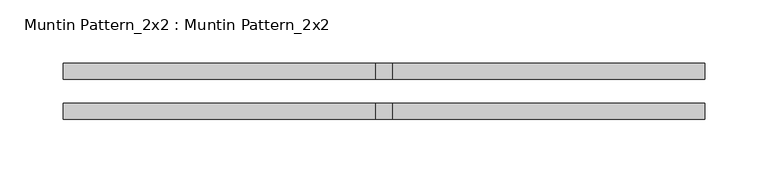
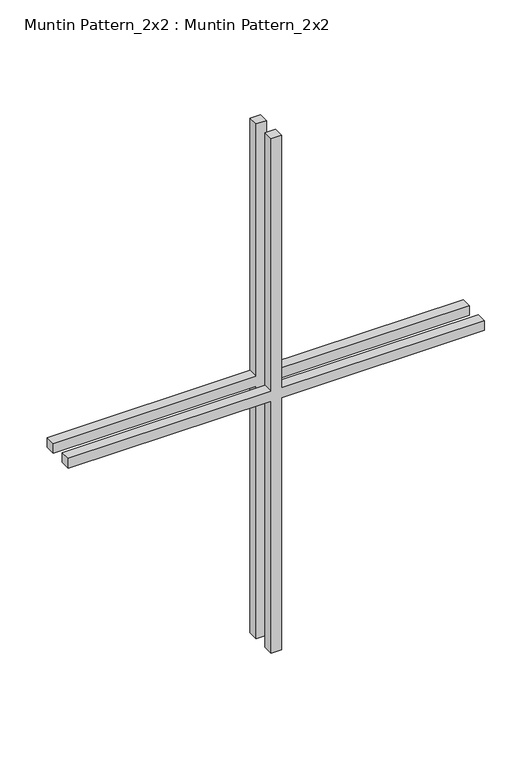
"""IFC4 building model written with IfcOpenShell, lengths in millimetres: proxy geometry, Muntin Pattern_2x2 : Muntin Pattern_2x2."""

from ifc_helpers import new_model, si_unit, frame, origin, place, context, project, spatial, polyline, outline, extrude, source, transform, mapped, element, save


def muntin_pattern_2x2_muntin_pattern_2x2_3eb6ceea(model_context):
    return source(origin(), model_context, "Body", "SweptSolid", [
        extrude(outline(polyline([(338.1375, -6.35), (338.1375, -254.0), (325.4375, -254.0), (325.4375, -6.35), (0.0, -6.35), (0.0, 6.35), (325.4375, 6.35), (325.4375, 254.0), (338.1375, 254.0), (338.1375, 6.35), (663.575, 6.35), (663.575, -6.35), (338.1375, -6.35)])), frame((0.0, -22.225, 0.0), z_axis=(0.0, 1.0, 0.0), x_axis=(0.0, 0.0, 1.0)), (0.0, 0.0, 1.0), 12.7),
        extrude(outline(polyline([(338.1375, -6.35), (338.1375, -254.0), (325.4375, -254.0), (325.4375, -6.35), (0.0, -6.35), (0.0, 6.35), (325.4375, 6.35), (325.4375, 254.0), (338.1375, 254.0), (338.1375, 6.35), (663.575, 6.35), (663.575, -6.35), (338.1375, -6.35)])), frame((0.0, 9.525, 0.0), z_axis=(0.0, 1.0, 0.0), x_axis=(0.0, 0.0, 1.0)), (0.0, 0.0, 1.0), 12.7),
    ])


if __name__ == "__main__":
    model = new_model("IFC4")
    model_context = context("Model", 3, world=origin())
    ifc_project = project(units=[si_unit("LENGTHUNIT", "METRE", prefix="MILLI")], contexts=[model_context])
    site = spatial("IfcSite", under=ifc_project)
    building = spatial("IfcBuilding", under=site)
    placement = place(None, origin())
    muntin_pattern_2x2_muntin_pattern_2x2_shape = muntin_pattern_2x2_muntin_pattern_2x2_3eb6ceea(model_context)
    element("IfcBuildingElementProxy", 1, Name="Muntin Pattern_2x2 : Muntin Pattern_2x2", ObjectType="Muntin Pattern_2x2 : Muntin Pattern_2x2", at=placement, inside=building, context=model_context, shape_type="MappedRepresentation", body=[
        mapped(muntin_pattern_2x2_muntin_pattern_2x2_shape, transform((0.0, 0.0, 0.0), x_axis=(1.0, 0.0, 0.0), y_axis=(0.0, 1.0, 0.0), z_axis=(0.0, 0.0, 1.0))),
    ])
    save(model, "model.ifc")

# Revit data of these elements
# Type "Muntin Pattern_2x2 : Muntin Pattern_2x2"
#   Width [instance default] = 4' - 0"
#   Thickness = 0' - 0 1/2"
#   Height [instance default] = 4' - 0"
#   Distance = 0' - 0 3/4"
#   Interior Material [instance default] = none
#   Exterior Material [instance default] = none
#   Default Elevation = 0
# Element 1 (IfcBuildingElementProxy, "Muntin Pattern_2x2 : Muntin Pattern_2x2")
#   Width = 1' - 8"
#   Height = 2' - 2 1/8"
#   Interior Material = Wood - Stained
#   Exterior Material = Clad - White
#   Materials on its faces: "Clad - White", "Wood - Stained"
# Materials
#   "Clad - White": class "Wood", colour RGB 242 242 238, transparency 0, Cost = 0
#   "Wood - Stained": class "Wood", colour RGB 224 178 126, transparency 0, Cost = 0
